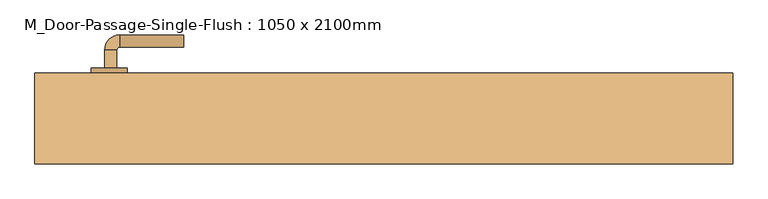
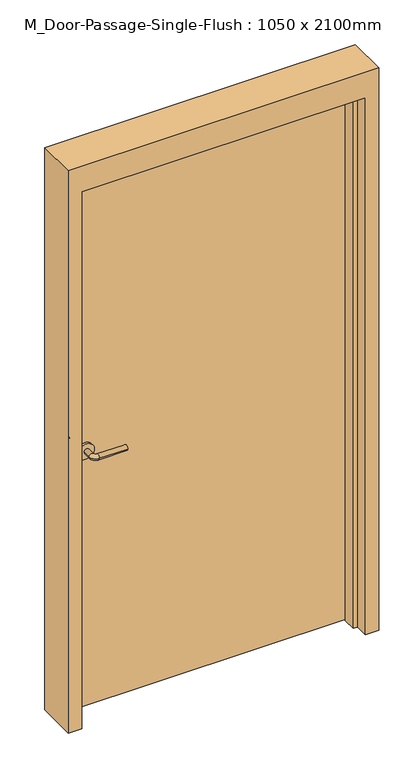
"""IFC4 building model written with IfcOpenShell, lengths in millimetres: door geometry, M_Door-Passage-Single-Flush : 1050 x 2100mm."""

from ifc_helpers import new_model, si_unit, point, frame, frame_2d, origin, origin_with_axes, place, context, project, spatial, polyline, circle_curve, ellipse_curve, trimmed, segment, composite_curve, outline, extrude, faceted_brep, source, transform, mapped, element, save
from ifc_brep_helpers import plane_surface, cylinder_surface, revolved_surface, advanced_brep


def m_door_passage_single_flush_1050_x_2100mm_780507da(model_context):
    return source(origin(), model_context, "Body", "SolidModel", [
        advanced_brep(
        [(-459.990625, 78.35, 1000.0), (-439.990625, 78.35, 1000.0), (-439.990625, 48.35, 1000.0), (-459.990625, 48.35, 1000.0), (-434.990625, 43.35, 1000.0), (-434.990625, 23.35, 1000.0), (-329.990625, 23.35, 1000.0), (-329.990625, 43.35, 1000.0)],
        [
            (0, 1, circle_curve(frame((-449.990625, 78.35, 1000.0), z_axis=(0.0, 1.0, 0.0), x_axis=(1.0, 0.0, 0.0)), 10.0)),
            (1, 0, circle_curve(frame((-449.990625, 78.35, 1000.0), z_axis=(0.0, 1.0, 0.0), x_axis=(1.0, 0.0, 0.0)), 10.0)),
            (1, 2),
            (2, 3, circle_curve(frame((-449.990625, 48.35, 1000.0), z_axis=(0.0, 1.0, 0.0), x_axis=(1.0, 0.0, 0.0)), 10.0)),
            (3, 0),
            (3, 2, circle_curve(frame((-449.990625, 48.35, 1000.0), z_axis=(0.0, 1.0, 0.0), x_axis=(1.0, 0.0, 0.0)), 10.0)),
            (4, 5, circle_curve(frame((-434.990625, 33.35, 1000.0), z_axis=(-1.0, 0.0, 0.0), x_axis=(0.0, 1.0, 0.0)), 10.0)),
            (5, 3, circle_curve(frame((-434.990625, 48.35, 1000.0), z_axis=(0.0, 0.0, -1.0), x_axis=(-1.0, 0.0, 0.0)), 25.0)),
            (2, 4, circle_curve(frame((-434.990625, 48.35, 1000.0), z_axis=(0.0, 0.0, 1.0), x_axis=(-1.0, 0.0, 0.0)), 5.0)),
            (5, 4, circle_curve(frame((-434.990625, 33.35, 1000.0), z_axis=(-1.0, 0.0, 0.0), x_axis=(0.0, 1.0, 0.0)), 10.0)),
            (6, 7, circle_curve(frame((-329.990625, 33.35, 1000.0), z_axis=(1.0, 0.0, 0.0), x_axis=(0.0, 1.0, 0.0)), 10.0)),
            (7, 6, circle_curve(frame((-329.990625, 33.35, 1000.0), z_axis=(1.0, 0.0, 0.0), x_axis=(0.0, 1.0, 0.0)), 10.0)),
            (4, 7),
            (6, 5),
        ],
        [
            plane_surface(frame((-449.990625, 78.35, 1000.0), z_axis=(0.0, 1.0, 0.0), x_axis=(0.0, 0.0, 1.0))),
            cylinder_surface(frame((-449.990625, 78.35, 1000.0), z_axis=(0.0, 1.0, 0.0), x_axis=(1.0, 0.0, 0.0)), 10.0),
            revolved_surface(trimmed(ellipse_curve(frame((-449.990625, 48.35, 1000.0), z_axis=(0.0, -1.0, 0.0), x_axis=(1.0, 0.0, 0.0)), 10.0, 10.0), [point((-459.990625, 48.35, 1000.0))], [point((-439.990625, 48.35, 1000.0))], True, "CARTESIAN"), (-434.990625, 48.35, 1000.0), (0.0, 0.0, -1.0)),
            revolved_surface(trimmed(ellipse_curve(frame((-449.990625, 48.35, 1000.0), z_axis=(0.0, -1.0, 0.0), x_axis=(1.0, 0.0, 0.0)), 10.0, 10.0), [point((-439.990625, 48.35, 1000.0))], [point((-459.990625, 48.35, 1000.0))], True, "CARTESIAN"), (-434.990625, 48.35, 1000.0), (0.0, 0.0, -1.0)),
            plane_surface(frame((-329.990625, 33.35, 1000.0), z_axis=(1.0, 0.0, 0.0), x_axis=(0.0, 0.0, 1.0))),
            cylinder_surface(frame((-434.990625, 33.35, 1000.0), z_axis=(-1.0, 0.0, 0.0), x_axis=(0.0, 1.0, 0.0)), 10.0),
        ],
        [
            (0, [[1, 2]]),
            (1, [[3, 4, 5, -2]]),
            (1, [[-5, 6, -3, -1]]),
            (2, [[7, 8, -4, 9]]),
            (3, [[10, -9, -6, -8]]),
            (4, [[11, 12]]),
            (5, [[13, -11, 14, -7]]),
            (5, [[-14, -12, -13, -10]]),
        ],
    ),
        extrude(outline(composite_curve([segment(trimmed(circle_curve(frame_2d((1000.0, -452.490625)), 30.0), [point((1000.0, -482.490625))], [point((1000.0, -422.490625))], False, "CARTESIAN"), True, "CONTINUOUS"), segment(trimmed(circle_curve(frame_2d((1000.0, -452.490625)), 30.0), [point((1000.0, -422.490625))], [point((1000.0, -482.490625))], False, "CARTESIAN"), True, "CONTINUOUS")], self_intersect=False)), frame((0.0, 78.35, 0.0), z_axis=(0.0, 1.0, 0.0), x_axis=(0.0, 0.0, 1.0)), (0.0, 0.0, 1.0), 8.0),
        advanced_brep(
        [(-459.990625, 139.35, 1000.0), (-439.990625, 139.35, 1000.0), (-459.990625, 169.35, 1000.0), (-439.990625, 169.35, 1000.0), (-434.990625, 174.35, 1000.0), (-434.990625, 194.35, 1000.0), (-329.990625, 194.35, 1000.0), (-329.990625, 174.35, 1000.0)],
        [
            (0, 1, circle_curve(frame((-449.990625, 139.35, 1000.0), z_axis=(0.0, -1.0, 0.0), x_axis=(1.0, 0.0, 0.0)), 10.0)),
            (1, 0, circle_curve(frame((-449.990625, 139.35, 1000.0), z_axis=(0.0, -1.0, 0.0), x_axis=(1.0, 0.0, 0.0)), 10.0)),
            (0, 2),
            (2, 3, circle_curve(frame((-449.990625, 169.35, 1000.0), z_axis=(0.0, -1.0, 0.0), x_axis=(1.0, 0.0, 0.0)), 10.0)),
            (3, 1),
            (3, 2, circle_curve(frame((-449.990625, 169.35, 1000.0), z_axis=(0.0, -1.0, 0.0), x_axis=(1.0, 0.0, 0.0)), 10.0)),
            (4, 3, circle_curve(frame((-434.990625, 169.35, 1000.0), z_axis=(0.0, 0.0, 1.0), x_axis=(-1.0, 0.0, 0.0)), 5.0)),
            (2, 5, circle_curve(frame((-434.990625, 169.35, 1000.0), z_axis=(0.0, 0.0, -1.0), x_axis=(-1.0, 0.0, 0.0)), 25.0)),
            (5, 4, circle_curve(frame((-434.990625, 184.35, 1000.0), z_axis=(-1.0, 0.0, 0.0), x_axis=(0.0, -1.0, 0.0)), 10.0)),
            (4, 5, circle_curve(frame((-434.990625, 184.35, 1000.0), z_axis=(-1.0, 0.0, 0.0), x_axis=(0.0, -1.0, 0.0)), 10.0)),
            (6, 7, circle_curve(frame((-329.990625, 184.35, 1000.0), z_axis=(1.0, 0.0, 0.0), x_axis=(0.0, -1.0, 0.0)), 10.0)),
            (7, 6, circle_curve(frame((-329.990625, 184.35, 1000.0), z_axis=(1.0, 0.0, 0.0), x_axis=(0.0, -1.0, 0.0)), 10.0)),
            (5, 6),
            (7, 4),
        ],
        [
            plane_surface(frame((-449.990625, 139.35, 1000.0), z_axis=(0.0, -1.0, 0.0), x_axis=(0.0, 0.0, 1.0))),
            cylinder_surface(frame((-449.990625, 139.35, 1000.0), z_axis=(0.0, -1.0, 0.0), x_axis=(1.0, 0.0, 0.0)), 10.0),
            revolved_surface(trimmed(ellipse_curve(frame((-449.990625, 169.35, 1000.0), z_axis=(0.0, -1.0, 0.0), x_axis=(1.0, 0.0, 0.0)), 10.0, 10.0), [point((-459.990625, 169.35, 1000.0))], [point((-439.990625, 169.35, 1000.0))], True, "CARTESIAN"), (-434.990625, 169.35, 1000.0), (0.0, 0.0, -1.0)),
            revolved_surface(trimmed(ellipse_curve(frame((-449.990625, 169.35, 1000.0), z_axis=(0.0, -1.0, 0.0), x_axis=(1.0, 0.0, 0.0)), 10.0, 10.0), [point((-439.990625, 169.35, 1000.0))], [point((-459.990625, 169.35, 1000.0))], True, "CARTESIAN"), (-434.990625, 169.35, 1000.0), (0.0, 0.0, -1.0)),
            plane_surface(frame((-329.990625, 184.35, 1000.0), z_axis=(1.0, 0.0, 0.0), x_axis=(0.0, 0.0, 1.0))),
            cylinder_surface(frame((-434.990625, 184.35, 1000.0), z_axis=(-1.0, 0.0, 0.0), x_axis=(0.0, -1.0, 0.0)), 10.0),
        ],
        [
            (0, [[1, 2]]),
            (1, [[-1, 3, 4, 5]]),
            (1, [[-2, -5, 6, -3]]),
            (2, [[7, -4, 8, 9]]),
            (3, [[-8, -6, -7, 10]]),
            (4, [[11, 12]]),
            (5, [[-9, 13, -12, 14]]),
            (5, [[-10, -14, -11, -13]]),
        ],
    ),
        extrude(outline(composite_curve([segment(trimmed(circle_curve(frame_2d((1000.0, -452.490625)), 30.0), [point((1000.0, -482.490625))], [point((1000.0, -422.490625))], False, "CARTESIAN"), True, "CONTINUOUS"), segment(trimmed(circle_curve(frame_2d((1000.0, -452.490625)), 30.0), [point((1000.0, -422.490625))], [point((1000.0, -482.490625))], False, "CARTESIAN"), True, "CONTINUOUS")], self_intersect=False)), frame((0.0, 131.35, 0.0), z_axis=(0.0, 1.0, 0.0), x_axis=(0.0, 0.0, 1.0)), (0.0, 0.0, 1.0), 8.0),
        faceted_brep([(525.0, 81.5875, 0.0), (525.0, 131.35, 0.0), (575.0, 131.35, 0.0), (575.0, -18.65, 0.0), (525.0, -18.65, 0.0), (525.0, 30.5625, 0.0), (509.125, 30.5625, 0.0), (509.125, 81.5875, 0.0), (525.0, 81.5875, 2100.0), (525.0, 131.35, 2100.0), (-525.0, 131.35, 2100.0), (-525.0, 131.35, 0.0), (-575.0, 131.35, 0.0), (-575.0, 131.35, 2200.0), (575.0, 131.35, 2200.0), (575.0, -18.65, 2200.0), (-575.0, -18.65, 2200.0), (-575.0, -18.65, 0.0), (-525.0, -18.65, 0.0), (-525.0, -18.65, 2100.0), (525.0, -18.65, 2100.0), (525.0, 30.5625, 2100.0), (-525.0, 30.5625, 2100.0), (-525.0, 30.5625, 0.0), (-509.125, 30.5625, 0.0), (-509.125, 30.5625, 2084.125), (509.125, 30.5625, 2084.125), (509.125, 81.5875, 2084.125), (-509.125, 81.5875, 2084.125), (-509.125, 81.5875, 0.0), (-525.0, 81.5875, 0.0), (-525.0, 81.5875, 2100.0)], [[[0, 1, 2, 3, 4, 5, 6, 7]], [[1, 0, 8, 9]], [[2, 1, 9, 10, 11, 12, 13, 14]], [[3, 2, 14, 15]], [[4, 3, 15, 16, 17, 18, 19, 20]], [[5, 4, 20, 21]], [[6, 5, 21, 22, 23, 24, 25, 26]], [[7, 6, 26, 27]], [[0, 7, 27, 28, 29, 30, 31, 8]], [[9, 8, 31, 10]], [[20, 19, 22, 21]], [[26, 25, 28, 27]], [[12, 11, 30, 29, 24, 23, 18, 17]], [[11, 10, 31, 30]], [[13, 12, 17, 16]], [[19, 18, 23, 22]], [[25, 24, 29, 28]], [[15, 14, 13, 16]]]),
        extrude(outline(polyline([(525.0, 86.35), (-525.0, 86.35), (-525.0, 131.35), (525.0, 131.35), (525.0, 86.35)])), origin_with_axes(), (0.0, 0.0, 1.0), 2100.0),
    ])


if __name__ == "__main__":
    model = new_model("IFC4")
    model_context = context("Model", 3, world=origin())
    ifc_project = project(units=[si_unit("LENGTHUNIT", "METRE", prefix="MILLI")], contexts=[model_context])
    site = spatial("IfcSite", under=ifc_project)
    building = spatial("IfcBuilding", under=site)
    placement = place(None, origin())
    m_door_passage_single_flush_1050_x_2100mm_shape = m_door_passage_single_flush_1050_x_2100mm_780507da(model_context)
    element("IfcDoor", 1, ObjectType="M_Door-Passage-Single-Flush : 1050 x 2100mm", at=placement, inside=building, context=model_context, shape_type="MappedRepresentation", body=[
        mapped(m_door_passage_single_flush_1050_x_2100mm_shape, transform((0.0, 0.0, 0.0), x_axis=(1.0, 0.0, 0.0), y_axis=(0.0, 1.0, 0.0), z_axis=(0.0, 0.0, 1.0))),
    ])
    save(model, "model.ifc")

# Revit data of these elements
# Type "M_Door-Passage-Single-Flush : 1050 x 2100mm"
#   Type Mark = "39"
#   Assembly Code = "B2030200"
#   Analytic Construction = "Wooden"
#   Thickness = 45 mm
#   Thermal Resistance (R) = 0.455703 (m²·K)/W
#   Swing Angle [instance default] = 90.00°
#   Strike Height = 1000 mm
#   Rough Width [instance default] = 1150 mm
#   Rough Height [instance default] = 2200 mm
#   MF Opening Height [instance default] = 100 mm
#   MF Opening Width [instance default] = 100 mm
#   Inset Calculate [instance default] = 105 mm
#   Masonry Inset [instance default] = 25 mm
#   Height = 2100 mm
#   Width = 1050 mm
#   Heat Transfer Coefficient (U) = 2.19465 W/(m²·K)
#   Masonry Frame Depth = 150 mm
#   Masonry Frame [instance default] = yes
#   Function = 1
#   Dry Wall Frame [instance default] = no
#   Panel Material = Wood - Birch
#   Frame Material = Metal - Paint Finish - Grey
#   Door Handle Material = Aluminum
#   Visual Light Transmittance = 0
#   Solar Heat Gain Coefficient = 0
#   Wall Closure = (empty or 0)
# Element 1 (IfcDoor, "M_Door-Passage-Single-Flush : 1050 x 2100mm")
#   Materials on its faces: "Aluminum", "Metal - Paint Finish - Grey", "Wood - Birch"
# Materials
#   "Wood - Birch": class "Wood", colour RGB 166 116 52, transparency 0, Cost = 0
#   "Metal - Paint Finish - Grey": class "Paint", colour RGB 104 104 104, transparency 0, Cost = 0
#   "Aluminum": class "Metal", colour RGB 244 244 244, transparency 0, Description = "Aluminum 6061", Cost = 0
